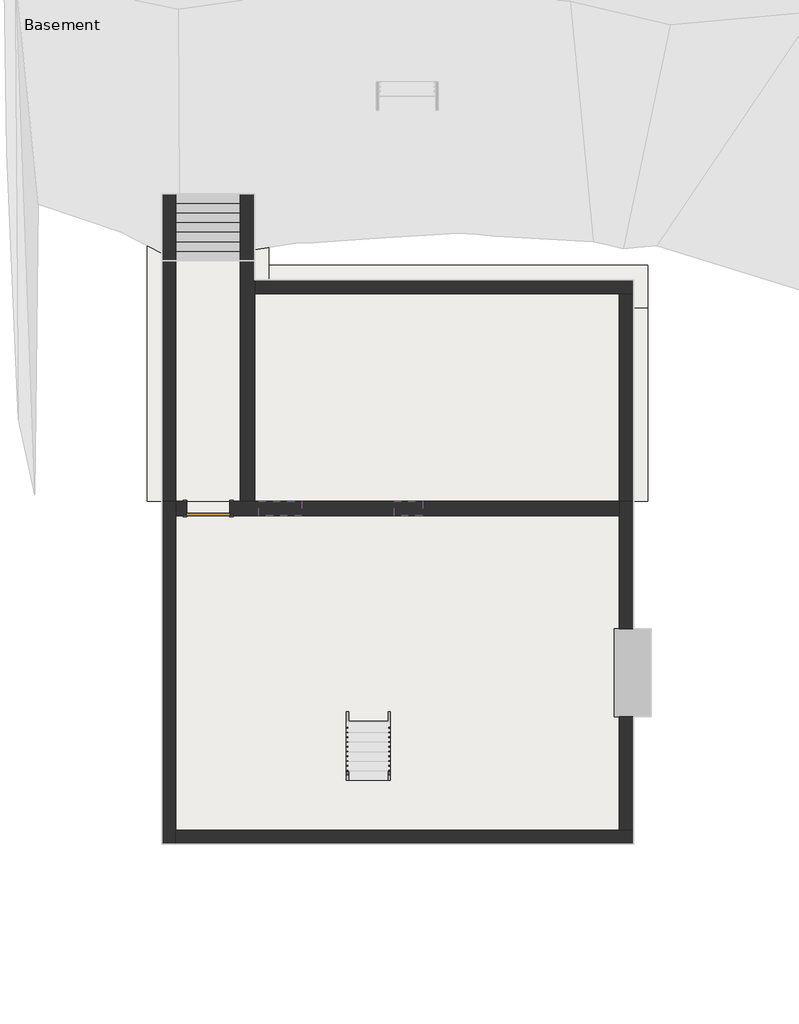
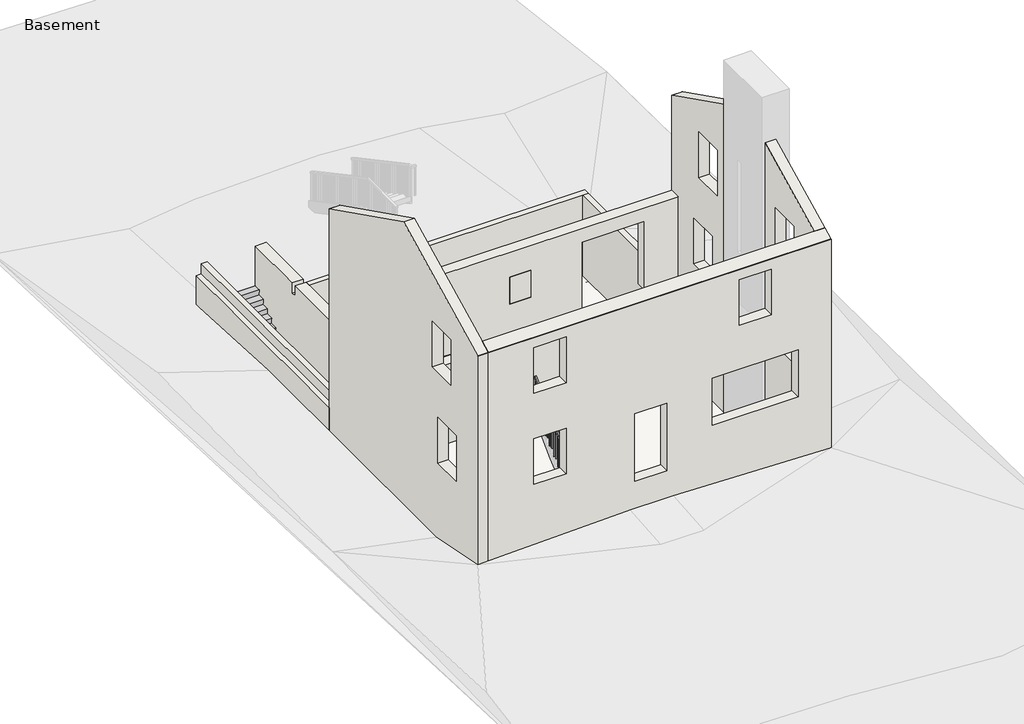
# One storey, part 1 of 2: 11 walls, 4 footings, 4 slabs, 2 railings, 1 door, 1 stair flight.
# Revit data of these elements (continued)
# Type "Single-Flush : 36\" x 84\"" (continued)
#   Visual Light Transmittance = 0
#   Solar Heat Gain Coefficient = 0
#   Function = (empty or 0)
#   Wall Closure = (empty or 0)
# Type "Bearing Footing - 36\" x 12\""
#   Assembly Code = "A1010110"
# Type "Handrail - Rectangular"
#   Assembly Code = "C2010400"
#   built-in parameter 1008612 = 0.0416667 (stored number, unit not read)
#   built-in parameter 1008611 = 0.0416667 (stored number, unit not read)
#   built-in parameter 1008609 = 0.333333 (stored number, unit not read)
#   built-in parameter 1008604 = 0.166667 (stored number, unit not read)
#   built-in parameter 1008603 = 0.166667 (stored number, unit not read)
#   Railing Height = 3' - 0"
#   built-in parameter 1008630 = 2
#   built-in parameter 1008610 = 2
#   built-in parameter 1008618 = Baluster - Square : 3/4"
# Type "4\" Concrete"
#   Assembly Code = "B1010"
#   Function = 0
#   Layers, outside or top first: 0' - 4" "Concrete, Lightweight" (function 1)
# Type "Pad 1"
#   Layers, outside or top first: 0' - 0 1/4" no material (function 1)
# Type "Foundation - 12\" Concrete"
#   Assembly Code = "A1010200"
#   Layers, outside or top first: 1' - 0" "Concrete, Cast-in-Place gray" (function 1)
# Type "Foundation - 12\" Concrete (w Brick Shelf)"
#   Assembly Code = "A1010200"
#   Layers, outside or top first: 1' - 0" "Concrete, Cast-in-Place gray" (function 1)
# Type "Generic - 12\""
#   Assembly Code = "B2010"
#   Layers, outside or top first: 1' - 0" no material (function 1)
# Element 1 (IfcDoor, "Single-Flush : 36\" x 84\"")
#   Phase Created = Existing
#   Materials on its faces: "Door - Frame", "Door - Panel"
# Elements 2, 5 (IfcFooting, "Bearing Footing - 36\" x 12\"")
#   Phase Created = New Construction
#   Materials on its faces: "Concrete, Cast-in-Place gray"
# Elements 3, 4 (IfcFooting, "Bearing Footing - 36\" x 12\"")
#   Comments = ""
#   Phase Created = New Construction
#   Materials on its faces: "Concrete, Cast-in-Place gray"
# Elements 6, 7 (IfcRailing, "Handrail - Rectangular")
#   Phase Created = Existing
# Element 8 (IfcSlab, "4\" Concrete")
#   built-in parameter 1001955 = 1.5708 (stored number, unit not read)
#   Height Offset From Level = 0' - 0"
#   Phase Created = New Construction
#   Materials on its faces: "Concrete, Lightweight"
# Elements 9, 10 (IfcSlab, "Pad 1")
#   built-in parameter 1012502 = -0.333333 (stored number, unit not read)
#   Phase Created = New Construction
# Element 11 (IfcSlab, "Pad 1")
#   built-in parameter 1012502 = -1.33333 (stored number, unit not read)
#   Phase Created = New Construction
# Element 12 (IfcStairFlight, "3/4\" Nosing")
#   Phase Created = New Construction
#   Materials on its faces: "Concrete, Cast-in-Place gray"
# Element 13 (IfcWall, "Foundation - 12\" Concrete")
#   built-in parameter 1001111 = -0' - 4"
#   Top Offset = 0' - 0"
#   Base Offset = -0' - 4"
#   wall height = 7' - 11 1/4"
#   Phase Created = New Construction
#   Base Constraint = Basement
#   Top Constraint = Top of Foundation
#   Materials on its faces: "Concrete, Cast-in-Place gray"
# Elements 14, 15, 16 (IfcWall, "Foundation - 12\" Concrete (w Brick Shelf)")
#   built-in parameter 1001111 = -0' - 4"
#   Top Offset = 0' - 0"
#   Base Offset = -0' - 4"
#   wall height = 7' - 11 1/4"
#   Phase Created = New Construction
#   Base Constraint = Basement
#   Top Constraint = Top of Foundation
#   Materials on its faces: "Concrete, Cast-in-Place gray"
# Element 17 (IfcWall, "Generic - 12\"")
#   Top Offset = 0' - 0"
#   Base Offset = 0' - 0"
#   wall height = 17' - 9"
#   Phase Created = Existing
#   Base Constraint = Basement
#   Top Constraint = Second Floor
#   Materials on its faces: "Default Wall"
# Elements 18, 19, 20, 21 (IfcWall, "Generic - 12\"")
#   Top Offset = 0' - 0"
#   Base Offset = 0' - 0"
#   wall height = 26' - 9"
#   Phase Created = Existing
#   Base Constraint = Basement
#   Top Constraint = Roof
#   Materials on its faces: "Default Wall"
# Elements 22, 23 (IfcWall, "Generic - 12\"")
#   Top Offset = 0' - 0"
#   Base Offset = 0' - 0"
#   Unconnected Height = 17' - 9"
#   wall height = 17' - 9"
#   Phase Created = New Construction
#   Base Constraint = Basement
#   Top Constraint = Basement
#   Materials on its faces: "Default Wall"
# Materials
#   "Door - Panel": class "Wood", colour RGB 210 159 95, transparency 0, Cost = 0
#   "Door - Frame": class "Miscellaneous", colour RGB 118 70 51, transparency 0, Cost = 0
#   "Concrete, Lightweight": class "Concrete", colour RGB 142 141 140, transparency 0, Description = "Lightweight concrete", Cost = 0
#   "Concrete, Cast-in-Place gray": class "Concrete", colour RGB 192 192 192, transparency 0, Description = "Cast-in-place concrete", Cost = 0
#   "Default Wall": class "Miscellaneous", colour RGB 128 128 128, transparency 0, Cost = 0
